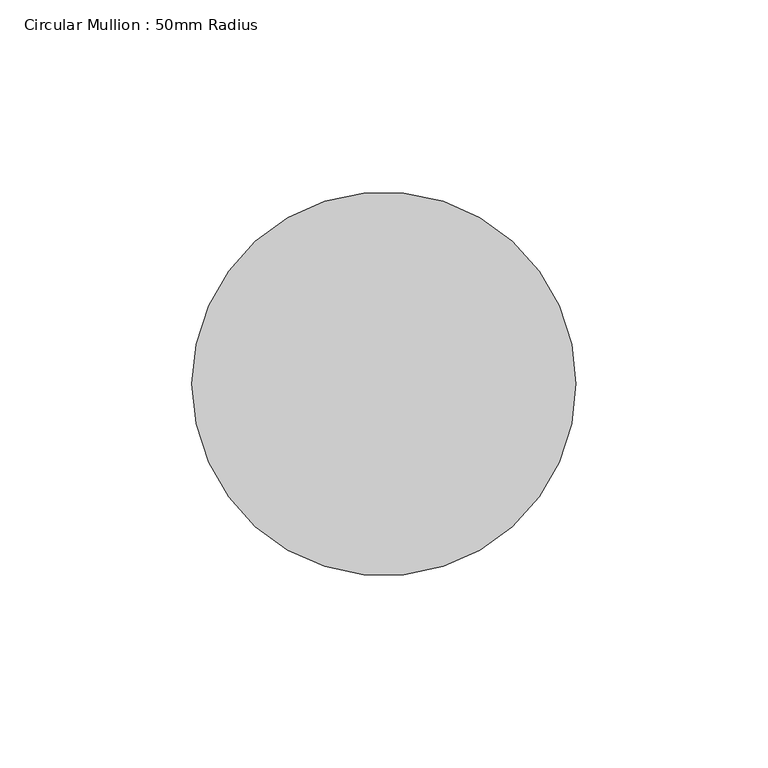
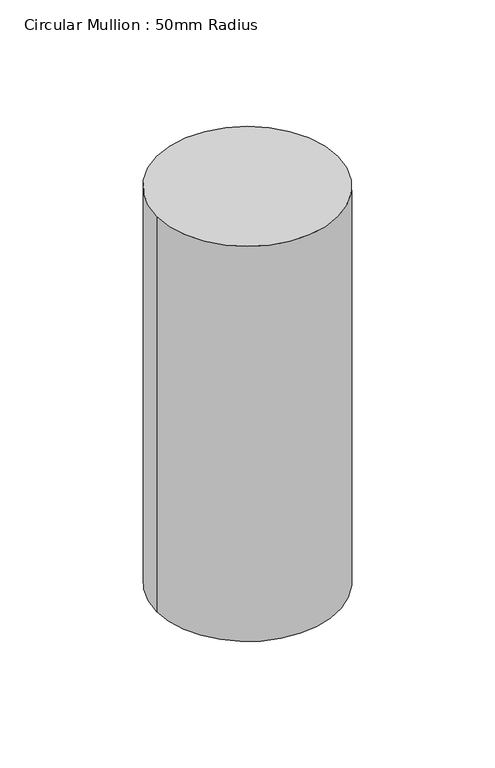
"""IFC4 building model written with IfcOpenShell, lengths in millimetres: member geometry, Circular Mullion : 50mm Radius."""

import ifcopenshell
import ifcopenshell.guid

model = None  # the IFC model being written
_history = None  # IfcOwnerHistory: only IFC2X3 demands one
_inside = {}  # id of a spatial element -> (the spatial element, [elements in it])
_under = {}  # id of a project, library or spatial element -> (it, [spatial elements below it])
_declared = {}  # id of a project -> (the project, [libraries it declares])
_typed = {}  # id of a type object -> (the type object, [elements of that type])
_made_of = {}  # id of a material, layer set ... -> (it, [elements and type objects made of it])


def new_model(schema):
    """Start an empty IFC model of exactly this schema.

    Asked for "IFC4X3", IfcOpenShell would pick the latest addendum, in which some entities
    have other attributes; the version numbers below select the first issue.
    IFC2X3 requires an IfcOwnerHistory on every rooted entity: one is made here for all.
    """
    global model, _history
    if schema == "IFC4X3":
        model = ifcopenshell.file(schema_version=(4, 3, 0, 0))
    else:
        model = ifcopenshell.file(schema=schema)
    _inside.clear()
    _under.clear()
    _declared.clear()
    _typed.clear()
    _made_of.clear()
    _history = None
    if model.schema == "IFC2X3":
        org = make("IfcOrganization", Name="unknown")
        user = make(
            "IfcPersonAndOrganization",
            ThePerson=make("IfcPerson", FamilyName="unknown"),
            TheOrganization=org,
        )
        app = make(
            "IfcApplication",
            ApplicationDeveloper=org,
            Version="unknown",
            ApplicationFullName="unknown",
            ApplicationIdentifier="unknown",
        )
        _history = make(
            "IfcOwnerHistory",
            OwningUser=user,
            OwningApplication=app,
            ChangeAction="ADDED",
            CreationDate=0,
        )
    return model


def make(cls, **values):
    """One entity of the class cls with the attributes given. An attribute that is None is left unset."""
    return model.create_entity(
        cls, **{name: value for name, value in values.items() if value is not None}
    )


def rooted(cls, **values):
    """An entity with a GlobalId (a new one), such as an element, a storey or a relation."""
    return make(cls, GlobalId=ifcopenshell.guid.new(), OwnerHistory=_history, **values)


def si_unit(unit_type, name, prefix=None):
    """IfcSIUnit, for example si_unit("LENGTHUNIT", "METRE", prefix="MILLI")."""
    return make("IfcSIUnit", UnitType=unit_type, Prefix=prefix, Name=name)


def assignment(units):
    """IfcUnitAssignment: the units of a project."""
    return None if units is None else make("IfcUnitAssignment", Units=units)


def point(xyz):
    """IfcCartesianPoint."""
    return None if xyz is None else make("IfcCartesianPoint", Coordinates=xyz)


def direction(xyz):
    """IfcDirection."""
    return None if xyz is None else make("IfcDirection", DirectionRatios=xyz)


def frame(location, z_axis=None, x_axis=None):
    """IfcAxis2Placement3D, a coordinate frame: its origin and axes. An axis left out is left unset."""
    return make(
        "IfcAxis2Placement3D",
        Location=point(location),
        Axis=direction(z_axis),
        RefDirection=direction(x_axis),
    )


def frame_2d(location, x_axis=None):
    """IfcAxis2Placement2D, a coordinate frame in the plane: its origin and x axis."""
    return make(
        "IfcAxis2Placement2D", Location=point(location), RefDirection=direction(x_axis)
    )


def origin():
    """The frame at (0, 0, 0) with its axes left unset."""
    return frame((0.0, 0.0, 0.0))


def origin_2d():
    """The frame at (0, 0) in the plane with its x axis left unset."""
    return frame_2d((0.0, 0.0))


def place(relative_to, where):
    """IfcLocalPlacement: puts the frame where relative to a parent placement (None: the world)."""
    return make(
        "IfcLocalPlacement", PlacementRelTo=relative_to, RelativePlacement=where
    )


def context(
    kind, dimensions, precision=None, world=None, true_north=None, identifier=None
):
    """IfcGeometricRepresentationContext, for example the 3D "Model" context."""
    return make(
        "IfcGeometricRepresentationContext",
        ContextIdentifier=identifier,
        ContextType=kind,
        CoordinateSpaceDimension=dimensions,
        Precision=precision,
        WorldCoordinateSystem=world,
        TrueNorth=true_north,
    )


def project(units=None, contexts=None):
    """IfcProject with its units and contexts."""
    return rooted(
        "IfcProject",
        Name="project",
        RepresentationContexts=contexts,
        UnitsInContext=assignment(units),
    )


def spatial(cls, under=None, at=None, **own):
    """A site, building, storey or space (cls), placed at a placement, below another one or the project."""
    s = rooted(cls, ObjectPlacement=at, **own)
    if under is not None:
        _under.setdefault(under.id(), (under, []))[1].append(s)
    return s


def circle_curve(where, radius):
    """IfcCircle in the frame where."""
    return make("IfcCircle", Position=where, Radius=radius)


def trimmed(basis, trim1, trim2, sense, master):
    """IfcTrimmedCurve: the piece of a basis curve between two trims."""
    return make(
        "IfcTrimmedCurve",
        BasisCurve=basis,
        Trim1=trim1,
        Trim2=trim2,
        SenseAgreement=sense,
        MasterRepresentation=master,
    )


def segment(curve, same_sense, transition):
    """IfcCompositeCurveSegment."""
    return make(
        "IfcCompositeCurveSegment",
        Transition=transition,
        SameSense=same_sense,
        ParentCurve=curve,
    )


def composite_curve(segments, self_intersect=None):
    """IfcCompositeCurve: segments joined end to end."""
    return make("IfcCompositeCurve", Segments=segments, SelfIntersect=self_intersect)


def outline(outer, holes=None, kind="AREA"):
    """IfcArbitraryClosedProfileDef: a profile drawn as a closed curve; with holes, ...WithVoids."""
    if holes is None:
        return make("IfcArbitraryClosedProfileDef", ProfileType=kind, OuterCurve=outer)
    return make(
        "IfcArbitraryProfileDefWithVoids",
        ProfileType=kind,
        OuterCurve=outer,
        InnerCurves=holes,
    )


def extrude(swept, where, along, depth):
    """IfcExtrudedAreaSolid: the profile swept, set in the frame where, extruded along a direction by depth."""
    return make(
        "IfcExtrudedAreaSolid",
        SweptArea=swept,
        Position=where,
        ExtrudedDirection=direction(along),
        Depth=depth,
    )


def shape(context_of_items, identifier, shape_type, items):
    """IfcShapeRepresentation: the items that make up one representation, for example the "Body"."""
    return make(
        "IfcShapeRepresentation",
        ContextOfItems=context_of_items,
        RepresentationIdentifier=identifier,
        RepresentationType=shape_type,
        Items=items,
    )


def source(mapping_origin, context_of_items, identifier, shape_type, items):
    """IfcRepresentationMap: a shape defined once, which mapped items show again and again."""
    return make(
        "IfcRepresentationMap",
        MappingOrigin=mapping_origin,
        MappedRepresentation=shape(context_of_items, identifier, shape_type, items),
    )


def transform(
    local_origin,
    x_axis=None,
    y_axis=None,
    z_axis=None,
    scale=None,
    scale2=None,
    scale3=None,
    uniform=True,
):
    """IfcCartesianTransformationOperator3D, or its non-uniform kind. x_axis, y_axis, z_axis: its Axis1, 2, 3."""
    if uniform:
        return make(
            "IfcCartesianTransformationOperator3D",
            Axis1=direction(x_axis),
            Axis2=direction(y_axis),
            LocalOrigin=point(local_origin),
            Scale=scale,
            Axis3=direction(z_axis),
        )
    return make(
        "IfcCartesianTransformationOperator3DnonUniform",
        Axis1=direction(x_axis),
        Axis2=direction(y_axis),
        LocalOrigin=point(local_origin),
        Scale=scale,
        Axis3=direction(z_axis),
        Scale2=scale2,
        Scale3=scale3,
    )


def mapped(mapping_source, mapping_target):
    """IfcMappedItem: shows the shape of a source again, moved by a transform."""
    return make(
        "IfcMappedItem", MappingSource=mapping_source, MappingTarget=mapping_target
    )


def made_of(thing, what):
    """Note that an element or type object is made of a material, layer set ...; save() writes the relation."""
    if what is not None:
        _made_of.setdefault(what.id(), (what, []))[1].append(thing)
    return thing


def element(
    cls,
    number,
    at=None,
    inside=None,
    cuts=None,
    type_object=None,
    material=None,
    context=None,
    identifier="Body",
    shape_type=None,
    held_by="IfcProductDefinitionShape",
    body=None,
    shapes=None,
    **own,
):
    """One element of the class cls, such as IfcWall. Its Tag is "e" and its number.

    at: its placement. inside: the storey or other place that contains it. cuts: it is an
    opening in that element (IfcRelVoidsElement). A single representation is given by context,
    identifier, shape_type and body (its items); several are given by shapes. held_by: the class
    of the entity that holds the representations. save() writes the other relations.
    """
    e = rooted(cls, Tag="e%d" % number, ObjectPlacement=at, **own)
    if body is not None:
        shapes = [shape(context, identifier, shape_type, body)]
    if shapes is not None:
        e.Representation = make(held_by, Representations=shapes)
    if inside is not None:
        _inside.setdefault(inside.id(), (inside, []))[1].append(e)
    if cuts is not None:
        rooted(
            "IfcRelVoidsElement", RelatingBuildingElement=cuts, RelatedOpeningElement=e
        )
    if type_object is not None:
        _typed.setdefault(type_object.id(), (type_object, []))[1].append(e)
    return made_of(e, material)


def aggregate(whole, parts):
    """IfcRelAggregates: a whole, such as a stair, and the parts it consists of."""
    return rooted("IfcRelAggregates", RelatingObject=whole, RelatedObjects=parts)


def save(model, path):
    """Write the relations noted so far, then the file.

    IfcRelAggregates (storeys below a building ...), IfcRelContainedInSpatialStructure (elements
    in a storey), IfcRelDefinesByType, IfcRelAssociatesMaterial and IfcRelDeclares: one each for
    every whole, place, type object, material and project.
    """
    for whole, parts in _under.values():
        aggregate(whole, parts)
    for where, things in _inside.values():
        rooted(
            "IfcRelContainedInSpatialStructure",
            RelatedElements=things,
            RelatingStructure=where,
        )
    for kind, things in _typed.values():
        rooted("IfcRelDefinesByType", RelatedObjects=things, RelatingType=kind)
    for what, things in _made_of.values():
        rooted("IfcRelAssociatesMaterial", RelatedObjects=things, RelatingMaterial=what)
    for by, libraries in _declared.values():
        rooted("IfcRelDeclares", RelatingContext=by, RelatedDefinitions=libraries)
    model.write(path)


def circular_mullion_50mm_radius_b038d907(model_context):
    return source(origin(), model_context, "Body", "SweptSolid", [
        extrude(outline(composite_curve([segment(trimmed(circle_curve(origin_2d(), 50.0), [point((50.0, 0.0))], [point((-50.0, 0.0))], False, "CARTESIAN"), True, "CONTINUOUS"), segment(trimmed(circle_curve(origin_2d(), 50.0), [point((-50.0, 0.0))], [point((50.0, 0.0))], False, "CARTESIAN"), True, "CONTINUOUS")], self_intersect=False)), frame((0.0, 0.0, -230.7098306), z_axis=(0.0, 0.0, 1.0), x_axis=(1.0, 0.0, 0.0)), (0.0, 0.0, 1.0), 230.7098306),
    ])


if __name__ == "__main__":
    model = new_model("IFC4")
    model_context = context("Model", 3, world=origin())
    ifc_project = project(units=[si_unit("LENGTHUNIT", "METRE", prefix="MILLI")], contexts=[model_context])
    site = spatial("IfcSite", under=ifc_project)
    building = spatial("IfcBuilding", under=site)
    placement = place(None, origin())
    circular_mullion_50mm_radius_shape = circular_mullion_50mm_radius_b038d907(model_context)
    element("IfcMember", 1, ObjectType="Circular Mullion : 50mm Radius", at=placement, inside=building, context=model_context, shape_type="MappedRepresentation", body=[
        mapped(circular_mullion_50mm_radius_shape, transform((0.0, 0.0, 0.0), x_axis=(1.0, 0.0, 0.0), y_axis=(0.0, 1.0, 0.0), z_axis=(0.0, 0.0, 1.0))),
    ])
    save(model, "model.ifc")

# Revit data of these elements
# Type "Circular Mullion : 50mm Radius"
#   built-in parameter 1007350 = 0.164042 (stored number, unit not read)
# Element 1 (IfcMember, "Circular Mullion : 50mm Radius")
#   Materials on its faces: "Aluminium"
# Materials
#   "Aluminium": class "Metal", colour RGB 247 247 247, transparency 0, Description = "Aluminium 6061", Cost = 0
